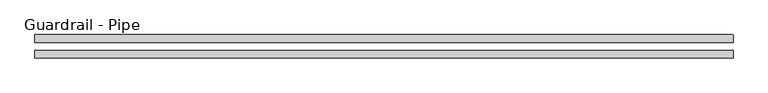
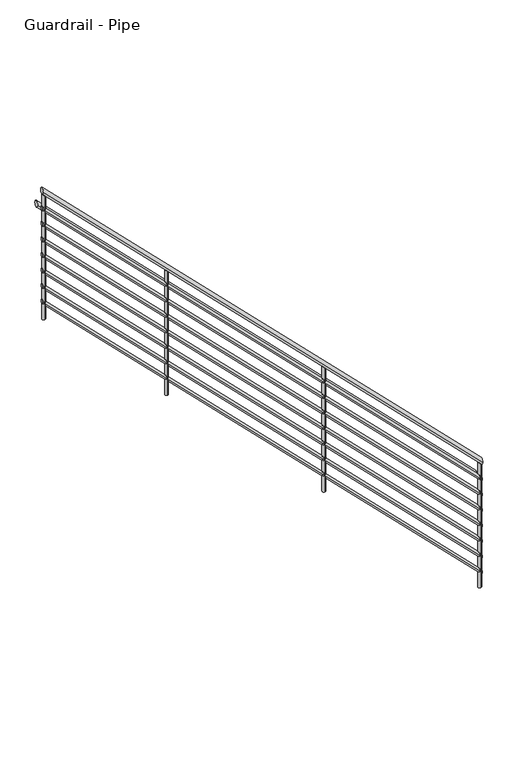
"""IFC4 building model written with IfcOpenShell, lengths in millimetres: railing geometry, Guardrail - Pipe."""

from ifc_helpers import new_model, si_unit, frame, origin, place, context, project, spatial, circle_curve, ellipse_curve, source, transform, mapped, element, save
from ifc_brep_helpers import plane_surface, cylinder_surface, advanced_brep


def guardrail_pipe_3270e9bd(model_context):
    return source(origin(), model_context, "Body", "AdvancedBrep", [
        advanced_brep(
        [(-7243.3085296, -4922.0836772, 1268.4592316), (-7243.3085296, -4960.1836772, 1268.4592316), (-10645.1029016, -4922.0836772, 4670.2536037), (-10645.1029016, -4960.1836772, 4670.2536037)],
        [
            (0, 1, ellipse_curve(frame((-7243.3085296, -4941.1336772, 1268.4592316), z_axis=(1.0, 0.0, 0.0), x_axis=(0.0, 0.0, -1.0)), 26.9407684, 19.05)),
            (1, 0, ellipse_curve(frame((-7243.3085296, -4941.1336772, 1268.4592316), z_axis=(1.0, 0.0, 0.0), x_axis=(0.0, 0.0, -1.0)), 26.9407684, 19.05)),
            (2, 3, ellipse_curve(frame((-10645.1029016, -4941.1336772, 4670.2536037), z_axis=(-1.0, 0.0, 0.0), x_axis=(0.0, 0.0, -1.0)), 26.9407684, 19.05)),
            (3, 2, ellipse_curve(frame((-10645.1029016, -4941.1336772, 4670.2536037), z_axis=(-1.0, 0.0, 0.0), x_axis=(0.0, 0.0, -1.0)), 26.9407684, 19.05)),
            (0, 2),
            (3, 1),
        ],
        [
            plane_surface(frame((-7243.3085296, -4941.1336772, 1295.4), z_axis=(1.0, 0.0, 0.0), x_axis=(0.0, -1.0, 0.0))),
            plane_surface(frame((-10645.1029016, -4941.1336772, 4697.194372), z_axis=(-1.0, 0.0, 0.0), x_axis=(0.0, -1.0, 0.0))),
            cylinder_surface(frame((-7256.7789137, -4941.1336772, 1281.9296158), z_axis=(0.7071067811865476, 0.0, -0.7071067811865476), x_axis=(0.0, -1.0, 0.0)), 19.05),
        ],
        [
            (0, [[1, 2]]),
            (1, [[3, 4]]),
            (2, [[-1, 5, -4, 6]]),
            (2, [[-2, -6, -3, -5]]),
        ],
    ),
        advanced_brep(
        [(-7243.3085296, -4928.4336772, 1125.0394878), (-7243.3085296, -4953.8336772, 1125.0394878), (-10645.1029016, -4928.4336772, 4526.8338598), (-10645.1029016, -4953.8336772, 4526.8338598)],
        [
            (0, 1, ellipse_curve(frame((-7243.3085296, -4941.1336772, 1125.0394878), z_axis=(1.0, 0.0, 0.0), x_axis=(0.0, 0.0, -1.0)), 17.9605122, 12.7)),
            (1, 0, ellipse_curve(frame((-7243.3085296, -4941.1336772, 1125.0394878), z_axis=(1.0, 0.0, 0.0), x_axis=(0.0, 0.0, -1.0)), 17.9605122, 12.7)),
            (2, 3, ellipse_curve(frame((-10645.1029016, -4941.1336772, 4526.8338598), z_axis=(-1.0, 0.0, 0.0), x_axis=(0.0, 0.0, -1.0)), 17.9605122, 12.7)),
            (3, 2, ellipse_curve(frame((-10645.1029016, -4941.1336772, 4526.8338598), z_axis=(-1.0, 0.0, 0.0), x_axis=(0.0, 0.0, -1.0)), 17.9605122, 12.7)),
            (0, 2),
            (3, 1),
        ],
        [
            plane_surface(frame((-7243.3085296, -4941.1336772, 1143.0), z_axis=(1.0, 0.0, 0.0), x_axis=(0.0, -1.0, 0.0))),
            plane_surface(frame((-10645.1029016, -4941.1336772, 4544.794372), z_axis=(-1.0, 0.0, 0.0), x_axis=(0.0, -1.0, 0.0))),
            cylinder_surface(frame((-7252.2887857, -4941.1336772, 1134.0197439), z_axis=(0.7071067811865476, 0.0, -0.7071067811865476), x_axis=(0.0, -1.0, 0.0)), 12.7),
        ],
        [
            (0, [[1, 2]]),
            (1, [[3, 4]]),
            (2, [[-1, 5, -4, 6]]),
            (2, [[-2, -6, -3, -5]]),
        ],
    ),
        advanced_brep(
        [(-7243.3085296, -4845.8836772, 1116.0592316), (-7243.3085296, -4883.9836772, 1116.0592316), (-10645.1029016, -4845.8836772, 4517.8536037), (-10645.1029016, -4883.9836772, 4517.8536037)],
        [
            (0, 1, ellipse_curve(frame((-7243.3085296, -4864.9336772, 1116.0592316), z_axis=(1.0, 0.0, 0.0), x_axis=(0.0, 0.0, -1.0)), 26.9407684, 19.05)),
            (1, 0, ellipse_curve(frame((-7243.3085296, -4864.9336772, 1116.0592316), z_axis=(1.0, 0.0, 0.0), x_axis=(0.0, 0.0, -1.0)), 26.9407684, 19.05)),
            (2, 3, ellipse_curve(frame((-10645.1029016, -4864.9336772, 4517.8536037), z_axis=(-1.0, 0.0, 0.0), x_axis=(0.0, 0.0, -1.0)), 26.9407684, 19.05)),
            (3, 2, ellipse_curve(frame((-10645.1029016, -4864.9336772, 4517.8536037), z_axis=(-1.0, 0.0, 0.0), x_axis=(0.0, 0.0, -1.0)), 26.9407684, 19.05)),
            (0, 2),
            (3, 1),
        ],
        [
            plane_surface(frame((-7243.3085296, -4864.9336772, 1143.0), z_axis=(1.0, 0.0, 0.0), x_axis=(0.0, -1.0, 0.0))),
            plane_surface(frame((-10645.1029016, -4864.9336772, 4544.794372), z_axis=(-1.0, 0.0, 0.0), x_axis=(0.0, -1.0, 0.0))),
            cylinder_surface(frame((-7256.7789137, -4864.9336772, 1129.5296158), z_axis=(0.7071067811865476, 0.0, -0.7071067811865476), x_axis=(0.0, -1.0, 0.0)), 19.05),
        ],
        [
            (0, [[1, 2]]),
            (1, [[3, 4]]),
            (2, [[-1, 5, -4, 6]]),
            (2, [[-2, -6, -3, -5]]),
        ],
    ),
        advanced_brep(
        [(-7243.3085296, -4928.4336772, 998.0394878), (-7243.3085296, -4953.8336772, 998.0394878), (-10645.1029016, -4928.4336772, 4399.8338598), (-10645.1029016, -4953.8336772, 4399.8338598)],
        [
            (0, 1, ellipse_curve(frame((-7243.3085296, -4941.1336772, 998.0394878), z_axis=(1.0, 0.0, 0.0), x_axis=(0.0, 0.0, -1.0)), 17.9605122, 12.7)),
            (1, 0, ellipse_curve(frame((-7243.3085296, -4941.1336772, 998.0394878), z_axis=(1.0, 0.0, 0.0), x_axis=(0.0, 0.0, -1.0)), 17.9605122, 12.7)),
            (2, 3, ellipse_curve(frame((-10645.1029016, -4941.1336772, 4399.8338598), z_axis=(-1.0, 0.0, 0.0), x_axis=(0.0, 0.0, -1.0)), 17.9605122, 12.7)),
            (3, 2, ellipse_curve(frame((-10645.1029016, -4941.1336772, 4399.8338598), z_axis=(-1.0, 0.0, 0.0), x_axis=(0.0, 0.0, -1.0)), 17.9605122, 12.7)),
            (0, 2),
            (3, 1),
        ],
        [
            plane_surface(frame((-7243.3085296, -4941.1336772, 1016.0), z_axis=(1.0, 0.0, 0.0), x_axis=(0.0, -1.0, 0.0))),
            plane_surface(frame((-10645.1029016, -4941.1336772, 4417.794372), z_axis=(-1.0, 0.0, 0.0), x_axis=(0.0, -1.0, 0.0))),
            cylinder_surface(frame((-7252.2887857, -4941.1336772, 1007.0197439), z_axis=(0.7071067811865476, 0.0, -0.7071067811865476), x_axis=(0.0, -1.0, 0.0)), 12.7),
        ],
        [
            (0, [[1, 2]]),
            (1, [[3, 4]]),
            (2, [[-1, 5, -4, 6]]),
            (2, [[-2, -6, -3, -5]]),
        ],
    ),
        advanced_brep(
        [(-7243.3085296, -4928.4336772, 871.0394878), (-7243.3085296, -4953.8336772, 871.0394878), (-10645.1029016, -4928.4336772, 4272.8338598), (-10645.1029016, -4953.8336772, 4272.8338598)],
        [
            (0, 1, ellipse_curve(frame((-7243.3085296, -4941.1336772, 871.0394878), z_axis=(1.0, 0.0, 0.0), x_axis=(0.0, 0.0, -1.0)), 17.9605122, 12.7)),
            (1, 0, ellipse_curve(frame((-7243.3085296, -4941.1336772, 871.0394878), z_axis=(1.0, 0.0, 0.0), x_axis=(0.0, 0.0, -1.0)), 17.9605122, 12.7)),
            (2, 3, ellipse_curve(frame((-10645.1029016, -4941.1336772, 4272.8338598), z_axis=(-1.0, 0.0, 0.0), x_axis=(0.0, 0.0, -1.0)), 17.9605122, 12.7)),
            (3, 2, ellipse_curve(frame((-10645.1029016, -4941.1336772, 4272.8338598), z_axis=(-1.0, 0.0, 0.0), x_axis=(0.0, 0.0, -1.0)), 17.9605122, 12.7)),
            (0, 2),
            (3, 1),
        ],
        [
            plane_surface(frame((-7243.3085296, -4941.1336772, 889.0), z_axis=(1.0, 0.0, 0.0), x_axis=(0.0, -1.0, 0.0))),
            plane_surface(frame((-10645.1029016, -4941.1336772, 4290.794372), z_axis=(-1.0, 0.0, 0.0), x_axis=(0.0, -1.0, 0.0))),
            cylinder_surface(frame((-7252.2887857, -4941.1336772, 880.0197439), z_axis=(0.7071067811865476, 0.0, -0.7071067811865476), x_axis=(0.0, -1.0, 0.0)), 12.7),
        ],
        [
            (0, [[1, 2]]),
            (1, [[3, 4]]),
            (2, [[-1, 5, -4, 6]]),
            (2, [[-2, -6, -3, -5]]),
        ],
    ),
        advanced_brep(
        [(-7243.3085296, -4928.4336772, 744.0394878), (-7243.3085296, -4953.8336772, 744.0394878), (-10645.1029016, -4928.4336772, 4145.8338598), (-10645.1029016, -4953.8336772, 4145.8338598)],
        [
            (0, 1, ellipse_curve(frame((-7243.3085296, -4941.1336772, 744.0394878), z_axis=(1.0, 0.0, 0.0), x_axis=(0.0, 0.0, -1.0)), 17.9605122, 12.7)),
            (1, 0, ellipse_curve(frame((-7243.3085296, -4941.1336772, 744.0394878), z_axis=(1.0, 0.0, 0.0), x_axis=(0.0, 0.0, -1.0)), 17.9605122, 12.7)),
            (2, 3, ellipse_curve(frame((-10645.1029016, -4941.1336772, 4145.8338598), z_axis=(-1.0, 0.0, 0.0), x_axis=(0.0, 0.0, -1.0)), 17.9605122, 12.7)),
            (3, 2, ellipse_curve(frame((-10645.1029016, -4941.1336772, 4145.8338598), z_axis=(-1.0, 0.0, 0.0), x_axis=(0.0, 0.0, -1.0)), 17.9605122, 12.7)),
            (0, 2),
            (3, 1),
        ],
        [
            plane_surface(frame((-7243.3085296, -4941.1336772, 762.0), z_axis=(1.0, 0.0, 0.0), x_axis=(0.0, -1.0, 0.0))),
            plane_surface(frame((-10645.1029016, -4941.1336772, 4163.794372), z_axis=(-1.0, 0.0, 0.0), x_axis=(0.0, -1.0, 0.0))),
            cylinder_surface(frame((-7252.2887857, -4941.1336772, 753.0197439), z_axis=(0.7071067811865476, 0.0, -0.7071067811865476), x_axis=(0.0, -1.0, 0.0)), 12.7),
        ],
        [
            (0, [[1, 2]]),
            (1, [[3, 4]]),
            (2, [[-1, 5, -4, 6]]),
            (2, [[-2, -6, -3, -5]]),
        ],
    ),
        advanced_brep(
        [(-7243.3085296, -4928.4336772, 617.0394878), (-7243.3085296, -4953.8336772, 617.0394878), (-10645.1029016, -4928.4336772, 4018.8338598), (-10645.1029016, -4953.8336772, 4018.8338598)],
        [
            (0, 1, ellipse_curve(frame((-7243.3085296, -4941.1336772, 617.0394878), z_axis=(1.0, 0.0, 0.0), x_axis=(0.0, 0.0, -1.0)), 17.9605122, 12.7)),
            (1, 0, ellipse_curve(frame((-7243.3085296, -4941.1336772, 617.0394878), z_axis=(1.0, 0.0, 0.0), x_axis=(0.0, 0.0, -1.0)), 17.9605122, 12.7)),
            (2, 3, ellipse_curve(frame((-10645.1029016, -4941.1336772, 4018.8338598), z_axis=(-1.0, 0.0, 0.0), x_axis=(0.0, 0.0, -1.0)), 17.9605122, 12.7)),
            (3, 2, ellipse_curve(frame((-10645.1029016, -4941.1336772, 4018.8338598), z_axis=(-1.0, 0.0, 0.0), x_axis=(0.0, 0.0, -1.0)), 17.9605122, 12.7)),
            (0, 2),
            (3, 1),
        ],
        [
            plane_surface(frame((-7243.3085296, -4941.1336772, 635.0), z_axis=(1.0, 0.0, 0.0), x_axis=(0.0, -1.0, 0.0))),
            plane_surface(frame((-10645.1029016, -4941.1336772, 4036.794372), z_axis=(-1.0, 0.0, 0.0), x_axis=(0.0, -1.0, 0.0))),
            cylinder_surface(frame((-7252.2887857, -4941.1336772, 626.0197439), z_axis=(0.7071067811865476, 0.0, -0.7071067811865476), x_axis=(0.0, -1.0, 0.0)), 12.7),
        ],
        [
            (0, [[1, 2]]),
            (1, [[3, 4]]),
            (2, [[-1, 5, -4, 6]]),
            (2, [[-2, -6, -3, -5]]),
        ],
    ),
        advanced_brep(
        [(-7243.3085296, -4928.4336772, 490.0394878), (-7243.3085296, -4953.8336772, 490.0394878), (-10645.1029016, -4928.4336772, 3891.8338598), (-10645.1029016, -4953.8336772, 3891.8338598)],
        [
            (0, 1, ellipse_curve(frame((-7243.3085296, -4941.1336772, 490.0394878), z_axis=(1.0, 0.0, 0.0), x_axis=(0.0, 0.0, -1.0)), 17.9605122, 12.7)),
            (1, 0, ellipse_curve(frame((-7243.3085296, -4941.1336772, 490.0394878), z_axis=(1.0, 0.0, 0.0), x_axis=(0.0, 0.0, -1.0)), 17.9605122, 12.7)),
            (2, 3, ellipse_curve(frame((-10645.1029016, -4941.1336772, 3891.8338598), z_axis=(-1.0, 0.0, 0.0), x_axis=(0.0, 0.0, -1.0)), 17.9605122, 12.7)),
            (3, 2, ellipse_curve(frame((-10645.1029016, -4941.1336772, 3891.8338598), z_axis=(-1.0, 0.0, 0.0), x_axis=(0.0, 0.0, -1.0)), 17.9605122, 12.7)),
            (0, 2),
            (3, 1),
        ],
        [
            plane_surface(frame((-7243.3085296, -4941.1336772, 508.0), z_axis=(1.0, 0.0, 0.0), x_axis=(0.0, -1.0, 0.0))),
            plane_surface(frame((-10645.1029016, -4941.1336772, 3909.794372), z_axis=(-1.0, 0.0, 0.0), x_axis=(0.0, -1.0, 0.0))),
            cylinder_surface(frame((-7252.2887857, -4941.1336772, 499.0197439), z_axis=(0.7071067811865476, 0.0, -0.7071067811865476), x_axis=(0.0, -1.0, 0.0)), 12.7),
        ],
        [
            (0, [[1, 2]]),
            (1, [[3, 4]]),
            (2, [[-1, 5, -4, 6]]),
            (2, [[-2, -6, -3, -5]]),
        ],
    ),
        advanced_brep(
        [(-7243.3085296, -4928.4336772, 363.0394878), (-7243.3085296, -4953.8336772, 363.0394878), (-10645.1029016, -4928.4336772, 3764.8338598), (-10645.1029016, -4953.8336772, 3764.8338598)],
        [
            (0, 1, ellipse_curve(frame((-7243.3085296, -4941.1336772, 363.0394878), z_axis=(1.0, 0.0, 0.0), x_axis=(0.0, 0.0, -1.0)), 17.9605122, 12.7)),
            (1, 0, ellipse_curve(frame((-7243.3085296, -4941.1336772, 363.0394878), z_axis=(1.0, 0.0, 0.0), x_axis=(0.0, 0.0, -1.0)), 17.9605122, 12.7)),
            (2, 3, ellipse_curve(frame((-10645.1029016, -4941.1336772, 3764.8338598), z_axis=(-1.0, 0.0, 0.0), x_axis=(0.0, 0.0, -1.0)), 17.9605122, 12.7)),
            (3, 2, ellipse_curve(frame((-10645.1029016, -4941.1336772, 3764.8338598), z_axis=(-1.0, 0.0, 0.0), x_axis=(0.0, 0.0, -1.0)), 17.9605122, 12.7)),
            (0, 2),
            (3, 1),
        ],
        [
            plane_surface(frame((-7243.3085296, -4941.1336772, 381.0), z_axis=(1.0, 0.0, 0.0), x_axis=(0.0, -1.0, 0.0))),
            plane_surface(frame((-10645.1029016, -4941.1336772, 3782.794372), z_axis=(-1.0, 0.0, 0.0), x_axis=(0.0, -1.0, 0.0))),
            cylinder_surface(frame((-7252.2887857, -4941.1336772, 372.0197439), z_axis=(0.7071067811865476, 0.0, -0.7071067811865476), x_axis=(0.0, -1.0, 0.0)), 12.7),
        ],
        [
            (0, [[1, 2]]),
            (1, [[3, 4]]),
            (2, [[-1, 5, -4, 6]]),
            (2, [[-2, -6, -3, -5]]),
        ],
    ),
        advanced_brep(
        [(-9681.7085296, -4953.8336772, 3679.9184633), (-9681.7085296, -4928.4336772, 3679.9184633), (-9681.7085296, -4928.4336772, 2667.0), (-9681.7085296, -4953.8336772, 2667.0)],
        [
            (0, 1, ellipse_curve(frame((-9681.7085296, -4941.1336772, 3679.9184633), z_axis=(-0.7071067811865471, 0.0, -0.7071067811865479), x_axis=(-0.7071067811865479, 0.0, 0.7071067811865471)), 17.9605122, 12.7)),
            (1, 2),
            (2, 3, circle_curve(frame((-9681.7085296, -4941.1336772, 2667.0), z_axis=(0.0, 0.0, 1.0), x_axis=(0.0, 1.0, 0.0)), 12.7)),
            (3, 0),
            (3, 2, circle_curve(frame((-9681.7085296, -4941.1336772, 2667.0), z_axis=(0.0, 0.0, 1.0), x_axis=(0.0, 1.0, 0.0)), 12.7)),
            (1, 0, ellipse_curve(frame((-9681.7085296, -4941.1336772, 3679.9184633), z_axis=(-0.7071067811865471, 0.0, -0.7071067811865479), x_axis=(-0.7071067811865479, 0.0, 0.7071067811865471)), 17.9605122, 12.7)),
        ],
        [
            cylinder_surface(frame((-9681.7085296, -4941.1336772, 2438.4), z_axis=(0.0, 0.0, 1.0), x_axis=(0.0, 1.0, 0.0)), 12.7),
            plane_surface(frame((-9707.1085296, -4915.7336772, 3705.3184633), z_axis=(0.7071067811865471, 0.0, 0.7071067811865479), x_axis=(0.0, -1.0, 0.0))),
            plane_surface(frame((-9656.3085296, -4915.7336772, 2667.0), z_axis=(0.0, 0.0, -1.0), x_axis=(0.0, -1.0, 0.0))),
        ],
        [
            (0, [[1, 2, 3, 4]]),
            (0, [[5, -2, 6, -4]]),
            (1, [[-6, -1]]),
            (2, [[-5, -3]]),
        ],
    ),
        advanced_brep(
        [(-8462.5085296, -4953.8336772, 2460.7184633), (-8462.5085296, -4928.4336772, 2460.7184633), (-8462.5085296, -4928.4336772, 1447.8), (-8462.5085296, -4953.8336772, 1447.8)],
        [
            (0, 1, ellipse_curve(frame((-8462.5085296, -4941.1336772, 2460.7184633), z_axis=(-0.7071067811865471, 0.0, -0.7071067811865479), x_axis=(-0.7071067811865479, 0.0, 0.7071067811865471)), 17.9605122, 12.7)),
            (1, 2),
            (2, 3, circle_curve(frame((-8462.5085296, -4941.1336772, 1447.8), z_axis=(0.0, 0.0, 1.0), x_axis=(0.0, 1.0, 0.0)), 12.7)),
            (3, 0),
            (3, 2, circle_curve(frame((-8462.5085296, -4941.1336772, 1447.8), z_axis=(0.0, 0.0, 1.0), x_axis=(0.0, 1.0, 0.0)), 12.7)),
            (1, 0, ellipse_curve(frame((-8462.5085296, -4941.1336772, 2460.7184633), z_axis=(-0.7071067811865471, 0.0, -0.7071067811865479), x_axis=(-0.7071067811865479, 0.0, 0.7071067811865471)), 17.9605122, 12.7)),
        ],
        [
            cylinder_surface(frame((-8462.5085296, -4941.1336772, 1219.2), z_axis=(0.0, 0.0, 1.0), x_axis=(0.0, 1.0, 0.0)), 12.7),
            plane_surface(frame((-8487.9085296, -4915.7336772, 2486.1184633), z_axis=(0.7071067811865471, 0.0, 0.7071067811865479), x_axis=(0.0, -1.0, 0.0))),
            plane_surface(frame((-8437.1085296, -4915.7336772, 1447.8), z_axis=(0.0, 0.0, -1.0), x_axis=(0.0, -1.0, 0.0))),
        ],
        [
            (0, [[1, 2, 3, 4]]),
            (0, [[5, -2, 6, -4]]),
            (1, [[-6, -1]]),
            (2, [[-5, -3]]),
        ],
    ),
        advanced_brep(
        [(-10632.4029016, -4953.8336772, 4630.6128353), (-10632.4029016, -4928.4336772, 4630.6128353), (-10632.4029016, -4928.4336772, 3617.694372), (-10632.4029016, -4953.8336772, 3617.694372)],
        [
            (0, 1, ellipse_curve(frame((-10632.4029016, -4941.1336772, 4630.6128353), z_axis=(-0.7071067811865471, 0.0, -0.7071067811865479), x_axis=(-0.7071067811865479, 0.0, 0.7071067811865471)), 17.9605122, 12.7)),
            (1, 2),
            (2, 3, circle_curve(frame((-10632.4029016, -4941.1336772, 3617.694372), z_axis=(0.0, 0.0, 1.0), x_axis=(0.0, 1.0, 0.0)), 12.7)),
            (3, 0),
            (3, 2, circle_curve(frame((-10632.4029016, -4941.1336772, 3617.694372), z_axis=(0.0, 0.0, 1.0), x_axis=(0.0, 1.0, 0.0)), 12.7)),
            (1, 0, ellipse_curve(frame((-10632.4029016, -4941.1336772, 4630.6128353), z_axis=(-0.7071067811865471, 0.0, -0.7071067811865479), x_axis=(-0.7071067811865479, 0.0, 0.7071067811865471)), 17.9605122, 12.7)),
        ],
        [
            cylinder_surface(frame((-10632.4029016, -4941.1336772, 3389.094372), z_axis=(0.0, 0.0, 1.0), x_axis=(0.0, 1.0, 0.0)), 12.7),
            plane_surface(frame((-10657.8029016, -4915.7336772, 4656.0128353), z_axis=(0.7071067811865471, 0.0, 0.7071067811865479), x_axis=(0.0, -1.0, 0.0))),
            plane_surface(frame((-10607.0029016, -4915.7336772, 3617.694372), z_axis=(0.0, 0.0, -1.0), x_axis=(0.0, -1.0, 0.0))),
        ],
        [
            (0, [[1, 2, 3, 4]]),
            (0, [[5, -2, 6, -4]]),
            (1, [[-6, -1]]),
            (2, [[-5, -3]]),
        ],
    ),
        advanced_brep(
        [(-7256.0085296, -4953.8336772, 1254.2184633), (-7256.0085296, -4928.4336772, 1254.2184633), (-7256.0085296, -4928.4336772, 241.3), (-7256.0085296, -4953.8336772, 241.3)],
        [
            (0, 1, ellipse_curve(frame((-7256.0085296, -4941.1336772, 1254.2184633), z_axis=(-0.7071067811865471, 0.0, -0.7071067811865479), x_axis=(-0.7071067811865479, 0.0, 0.7071067811865471)), 17.9605122, 12.7)),
            (1, 2),
            (2, 3, circle_curve(frame((-7256.0085296, -4941.1336772, 241.3), z_axis=(0.0, 0.0, 1.0), x_axis=(0.0, 1.0, 0.0)), 12.7)),
            (3, 0),
            (3, 2, circle_curve(frame((-7256.0085296, -4941.1336772, 241.3), z_axis=(0.0, 0.0, 1.0), x_axis=(0.0, 1.0, 0.0)), 12.7)),
            (1, 0, ellipse_curve(frame((-7256.0085296, -4941.1336772, 1254.2184633), z_axis=(-0.7071067811865471, 0.0, -0.7071067811865479), x_axis=(-0.7071067811865479, 0.0, 0.7071067811865471)), 17.9605122, 12.7)),
        ],
        [
            cylinder_surface(frame((-7256.0085296, -4941.1336772, 12.7), z_axis=(0.0, 0.0, 1.0), x_axis=(0.0, 1.0, 0.0)), 12.7),
            plane_surface(frame((-7281.4085296, -4915.7336772, 1279.6184633), z_axis=(0.7071067811865471, 0.0, 0.7071067811865479), x_axis=(0.0, -1.0, 0.0))),
            plane_surface(frame((-7230.6085296, -4915.7336772, 241.3), z_axis=(0.0, 0.0, -1.0), x_axis=(0.0, -1.0, 0.0))),
        ],
        [
            (0, [[1, 2, 3, 4]]),
            (0, [[5, -2, 6, -4]]),
            (1, [[-6, -1]]),
            (2, [[-5, -3]]),
        ],
    ),
    ])


if __name__ == "__main__":
    model = new_model("IFC4")
    model_context = context("Model", 3, world=origin())
    ifc_project = project(units=[si_unit("LENGTHUNIT", "METRE", prefix="MILLI")], contexts=[model_context])
    site = spatial("IfcSite", under=ifc_project)
    building = spatial("IfcBuilding", under=site)
    placement = place(None, origin())
    guardrail_pipe_shape = guardrail_pipe_3270e9bd(model_context)
    element("IfcRailing", 1, ObjectType="Guardrail - Pipe", at=placement, inside=building, context=model_context, shape_type="MappedRepresentation", body=[
        mapped(guardrail_pipe_shape, transform((0.0, 0.0, 0.0), x_axis=(1.0, 0.0, 0.0), y_axis=(0.0, 1.0, 0.0), z_axis=(0.0, 0.0, 1.0))),
    ])
    save(model, "model.ifc")

# Revit data of these elements
# Element 1 (IfcRailing, "Guardrail - Pipe")
#   Materials on its faces: "Plastic - Vinyl Cove Base"
# Materials
#   "Plastic - Vinyl Cove Base": class "Plastic", colour RGB 5 5 5, transparency 0, Cost = 0
